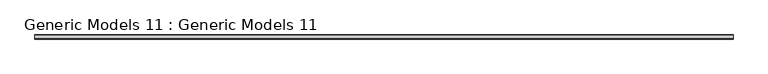
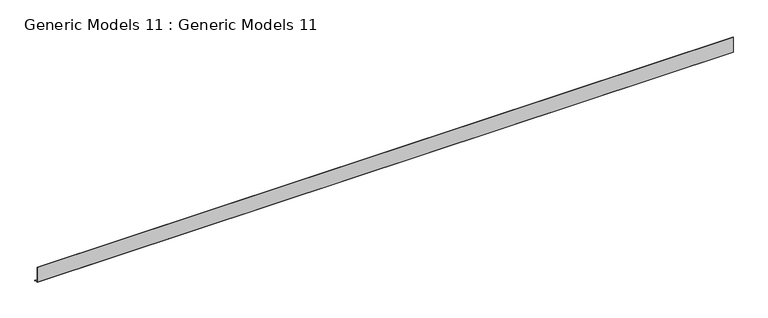
"""IFC4 building model written with IfcOpenShell, lengths in millimetres: proxy geometry, Generic Models 11 : Generic Models 11."""

from ifc_helpers import new_model, si_unit, frame, origin, place, context, project, spatial, polyline, outline, extrude, source, transform, mapped, element, save


def generic_models_11_generic_models_11_f55eb675(model_context):
    return source(origin(), model_context, "Body", "SweptSolid", [
        extrude(outline(polyline([(40954.6606612, 269266.19375), (40954.6606612, 269398.75), (40956.2481612, 269398.75), (40956.2481612, 269267.78125), (40983.8932252, 269267.78125), (40988.3833533, 269263.2911219), (40987.2608213, 269262.1685899), (40983.2356612, 269266.19375), (40954.6606612, 269266.19375)])), frame((26424.3233872, 0.0, 0.0), z_axis=(1.0, 0.0, 0.0), x_axis=(0.0, 1.0, 0.0)), (0.0, 0.0, 1.0), 5752.7106906),
    ])


if __name__ == "__main__":
    model = new_model("IFC4")
    model_context = context("Model", 3, world=origin())
    ifc_project = project(units=[si_unit("LENGTHUNIT", "METRE", prefix="MILLI")], contexts=[model_context])
    site = spatial("IfcSite", under=ifc_project)
    building = spatial("IfcBuilding", under=site)
    placement = place(None, origin())
    generic_models_11_generic_models_11_shape = generic_models_11_generic_models_11_f55eb675(model_context)
    element("IfcBuildingElementProxy", 1, Name="Generic Models 11 : Generic Models 11", ObjectType="Generic Models 11 : Generic Models 11", at=placement, inside=building, context=model_context, shape_type="MappedRepresentation", body=[
        mapped(generic_models_11_generic_models_11_shape, transform((0.0, 0.0, 0.0), x_axis=(1.0, 0.0, 0.0), y_axis=(0.0, 1.0, 0.0), z_axis=(0.0, 0.0, 1.0))),
    ])
    save(model, "model.ifc")

# Revit data of these elements
# Element 1 (IfcBuildingElementProxy, "Generic Models 11 : Generic Models 11")
#   Materials on its faces: "GALV. BRAKE METAL - (COLOR: DARK BRONZE)"
# Materials
#   "GALV. BRAKE METAL - (COLOR: DARK BRONZE)": class "Generic", colour RGB 72 52 47, transparency 0, Cost = 0
